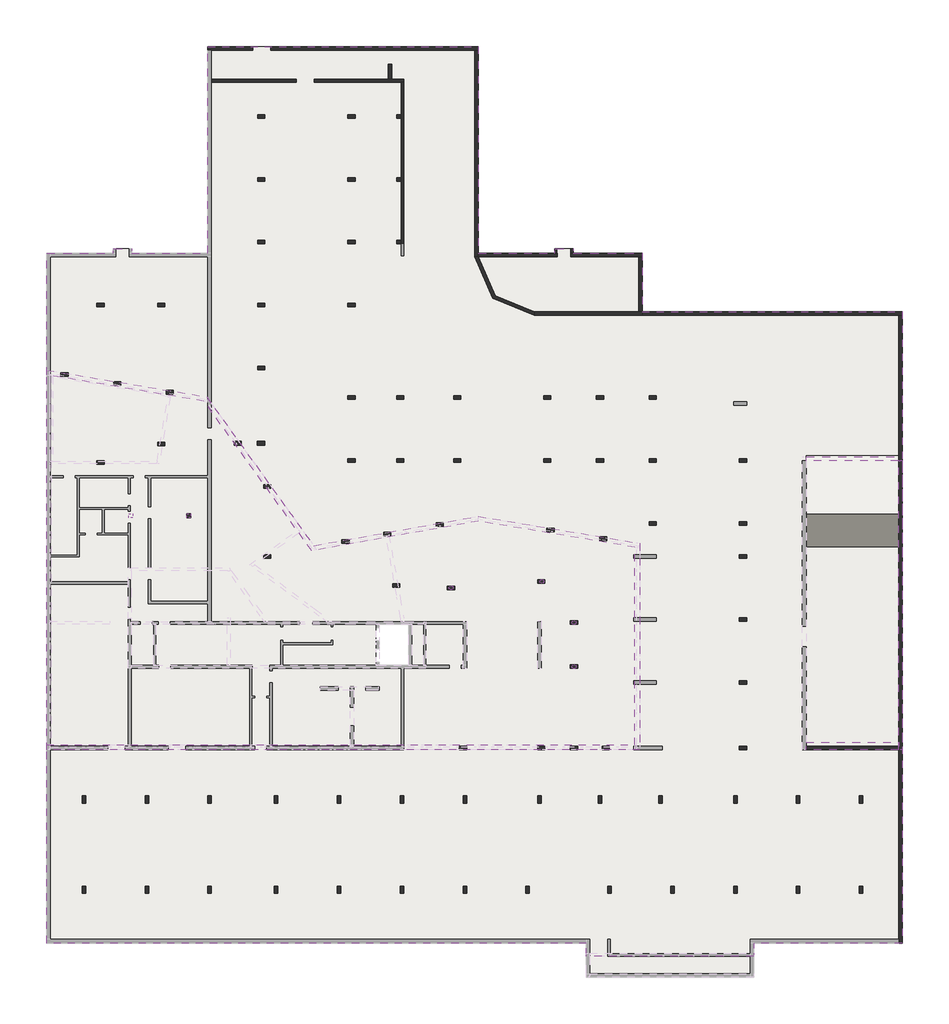
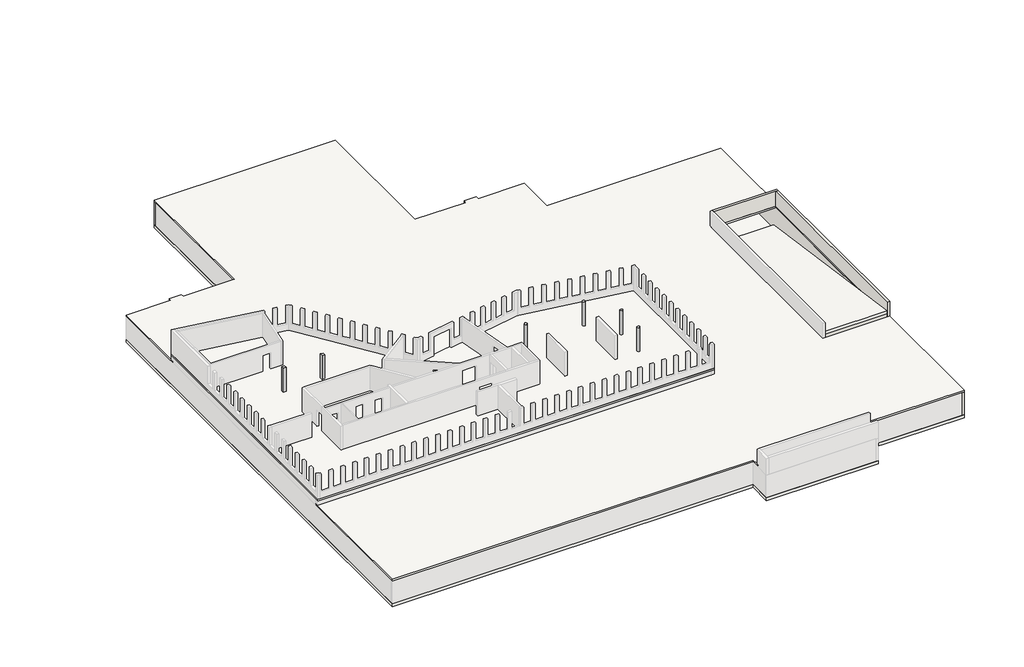
# One storey, part 4 of 4: 89 columns, 17 walls, 4 slabs.
"""IFC4 building model written with IfcOpenShell, lengths in millimetres."""

import ifcopenshell
import ifcopenshell.guid

model = None  # the IFC model being written
_history = None  # IfcOwnerHistory: only IFC2X3 demands one
_inside = {}  # id of a spatial element -> (the spatial element, [elements in it])
_under = {}  # id of a project, library or spatial element -> (it, [spatial elements below it])
_declared = {}  # id of a project -> (the project, [libraries it declares])
_typed = {}  # id of a type object -> (the type object, [elements of that type])
_made_of = {}  # id of a material, layer set ... -> (it, [elements and type objects made of it])


def new_model(schema):
    """Start an empty IFC model of exactly this schema.

    Asked for "IFC4X3", IfcOpenShell would pick the latest addendum, in which some entities
    have other attributes; the version numbers below select the first issue.
    IFC2X3 requires an IfcOwnerHistory on every rooted entity: one is made here for all.
    """
    global model, _history
    if schema == "IFC4X3":
        model = ifcopenshell.file(schema_version=(4, 3, 0, 0))
    else:
        model = ifcopenshell.file(schema=schema)
    _inside.clear()
    _under.clear()
    _declared.clear()
    _typed.clear()
    _made_of.clear()
    _history = None
    if model.schema == "IFC2X3":
        org = make("IfcOrganization", Name="unknown")
        user = make(
            "IfcPersonAndOrganization",
            ThePerson=make("IfcPerson", FamilyName="unknown"),
            TheOrganization=org,
        )
        app = make(
            "IfcApplication",
            ApplicationDeveloper=org,
            Version="unknown",
            ApplicationFullName="unknown",
            ApplicationIdentifier="unknown",
        )
        _history = make(
            "IfcOwnerHistory",
            OwningUser=user,
            OwningApplication=app,
            ChangeAction="ADDED",
            CreationDate=0,
        )
    return model


def make(cls, **values):
    """One entity of the class cls with the attributes given. An attribute that is None is left unset."""
    return model.create_entity(
        cls, **{name: value for name, value in values.items() if value is not None}
    )


def rooted(cls, **values):
    """An entity with a GlobalId (a new one), such as an element, a storey or a relation."""
    return make(cls, GlobalId=ifcopenshell.guid.new(), OwnerHistory=_history, **values)


def si_unit(unit_type, name, prefix=None):
    """IfcSIUnit, for example si_unit("LENGTHUNIT", "METRE", prefix="MILLI")."""
    return make("IfcSIUnit", UnitType=unit_type, Prefix=prefix, Name=name)


def assignment(units):
    """IfcUnitAssignment: the units of a project."""
    return None if units is None else make("IfcUnitAssignment", Units=units)


def point(xyz):
    """IfcCartesianPoint."""
    return None if xyz is None else make("IfcCartesianPoint", Coordinates=xyz)


def direction(xyz):
    """IfcDirection."""
    return None if xyz is None else make("IfcDirection", DirectionRatios=xyz)


def frame(location, z_axis=None, x_axis=None):
    """IfcAxis2Placement3D, a coordinate frame: its origin and axes. An axis left out is left unset."""
    return make(
        "IfcAxis2Placement3D",
        Location=point(location),
        Axis=direction(z_axis),
        RefDirection=direction(x_axis),
    )


def frame_2d(location, x_axis=None):
    """IfcAxis2Placement2D, a coordinate frame in the plane: its origin and x axis."""
    return make(
        "IfcAxis2Placement2D", Location=point(location), RefDirection=direction(x_axis)
    )


def origin():
    """The frame at (0, 0, 0) with its axes left unset."""
    return frame((0.0, 0.0, 0.0))


def place(relative_to, where):
    """IfcLocalPlacement: puts the frame where relative to a parent placement (None: the world)."""
    return make(
        "IfcLocalPlacement", PlacementRelTo=relative_to, RelativePlacement=where
    )


def context(
    kind, dimensions, precision=None, world=None, true_north=None, identifier=None
):
    """IfcGeometricRepresentationContext, for example the 3D "Model" context."""
    return make(
        "IfcGeometricRepresentationContext",
        ContextIdentifier=identifier,
        ContextType=kind,
        CoordinateSpaceDimension=dimensions,
        Precision=precision,
        WorldCoordinateSystem=world,
        TrueNorth=true_north,
    )


def project(units=None, contexts=None):
    """IfcProject with its units and contexts."""
    return rooted(
        "IfcProject",
        Name="project",
        RepresentationContexts=contexts,
        UnitsInContext=assignment(units),
    )


def spatial(cls, under=None, at=None, **own):
    """A site, building, storey or space (cls), placed at a placement, below another one or the project."""
    s = rooted(cls, ObjectPlacement=at, **own)
    if under is not None:
        _under.setdefault(under.id(), (under, []))[1].append(s)
    return s


def polyline(points):
    """IfcPolyline through the points."""
    return make("IfcPolyline", Points=[point(p) for p in points])


def circle_curve(where, radius):
    """IfcCircle in the frame where."""
    return make("IfcCircle", Position=where, Radius=radius)


def trimmed(basis, trim1, trim2, sense, master):
    """IfcTrimmedCurve: the piece of a basis curve between two trims."""
    return make(
        "IfcTrimmedCurve",
        BasisCurve=basis,
        Trim1=trim1,
        Trim2=trim2,
        SenseAgreement=sense,
        MasterRepresentation=master,
    )


def segment(curve, same_sense, transition):
    """IfcCompositeCurveSegment."""
    return make(
        "IfcCompositeCurveSegment",
        Transition=transition,
        SameSense=same_sense,
        ParentCurve=curve,
    )


def composite_curve(segments, self_intersect=None):
    """IfcCompositeCurve: segments joined end to end."""
    return make("IfcCompositeCurve", Segments=segments, SelfIntersect=self_intersect)


def outline(outer, holes=None, kind="AREA"):
    """IfcArbitraryClosedProfileDef: a profile drawn as a closed curve; with holes, ...WithVoids."""
    if holes is None:
        return make("IfcArbitraryClosedProfileDef", ProfileType=kind, OuterCurve=outer)
    return make(
        "IfcArbitraryProfileDefWithVoids",
        ProfileType=kind,
        OuterCurve=outer,
        InnerCurves=holes,
    )


def extrude(swept, where, along, depth):
    """IfcExtrudedAreaSolid: the profile swept, set in the frame where, extruded along a direction by depth."""
    return make(
        "IfcExtrudedAreaSolid",
        SweptArea=swept,
        Position=where,
        ExtrudedDirection=direction(along),
        Depth=depth,
    )


def faces_of(points, faces, orient=None, outer=None):
    """IfcFace entities. A face is a list of loops; a loop is a list of indices into points, from 0.

    orient and outer hold one flag for each loop. By default every Orientation is true, the
    first loop of a face is its IfcFaceOuterBound and the others are IfcFaceBound.
    """
    made = []
    for i, loops in enumerate(faces):
        bounds = []
        for j, loop in enumerate(loops):
            is_outer = j == 0 if outer is None else outer[i][j]
            bounds.append(
                make(
                    "IfcFaceOuterBound" if is_outer else "IfcFaceBound",
                    Bound=make("IfcPolyLoop", Polygon=[points[k] for k in loop]),
                    Orientation=True if orient is None else orient[i][j],
                )
            )
        made.append(make("IfcFace", Bounds=bounds))
    return made


def faceted_brep(points, faces, orient=None, outer=None, voids=None):
    """IfcFacetedBrep: a solid bounded by flat faces; with voids (closed shells), ...WithVoids."""
    shared = [point(p) for p in points]
    hull = make("IfcClosedShell", CfsFaces=faces_of(shared, faces, orient, outer))
    if voids is None:
        return make("IfcFacetedBrep", Outer=hull)
    return make(
        "IfcFacetedBrepWithVoids",
        Outer=hull,
        Voids=[
            make(cls, CfsFaces=faces_of(shared, fs, o, b)) for cls, fs, o, b in voids
        ],
    )


def shape(context_of_items, identifier, shape_type, items):
    """IfcShapeRepresentation: the items that make up one representation, for example the "Body"."""
    return make(
        "IfcShapeRepresentation",
        ContextOfItems=context_of_items,
        RepresentationIdentifier=identifier,
        RepresentationType=shape_type,
        Items=items,
    )


def source(mapping_origin, context_of_items, identifier, shape_type, items):
    """IfcRepresentationMap: a shape defined once, which mapped items show again and again."""
    return make(
        "IfcRepresentationMap",
        MappingOrigin=mapping_origin,
        MappedRepresentation=shape(context_of_items, identifier, shape_type, items),
    )


def transform(
    local_origin,
    x_axis=None,
    y_axis=None,
    z_axis=None,
    scale=None,
    scale2=None,
    scale3=None,
    uniform=True,
):
    """IfcCartesianTransformationOperator3D, or its non-uniform kind. x_axis, y_axis, z_axis: its Axis1, 2, 3."""
    if uniform:
        return make(
            "IfcCartesianTransformationOperator3D",
            Axis1=direction(x_axis),
            Axis2=direction(y_axis),
            LocalOrigin=point(local_origin),
            Scale=scale,
            Axis3=direction(z_axis),
        )
    return make(
        "IfcCartesianTransformationOperator3DnonUniform",
        Axis1=direction(x_axis),
        Axis2=direction(y_axis),
        LocalOrigin=point(local_origin),
        Scale=scale,
        Axis3=direction(z_axis),
        Scale2=scale2,
        Scale3=scale3,
    )


def mapped(mapping_source, mapping_target):
    """IfcMappedItem: shows the shape of a source again, moved by a transform."""
    return make(
        "IfcMappedItem", MappingSource=mapping_source, MappingTarget=mapping_target
    )


def made_of(thing, what):
    """Note that an element or type object is made of a material, layer set ...; save() writes the relation."""
    if what is not None:
        _made_of.setdefault(what.id(), (what, []))[1].append(thing)
    return thing


def element(
    cls,
    number,
    at=None,
    inside=None,
    cuts=None,
    type_object=None,
    material=None,
    context=None,
    identifier="Body",
    shape_type=None,
    held_by="IfcProductDefinitionShape",
    body=None,
    shapes=None,
    **own,
):
    """One element of the class cls, such as IfcWall. Its Tag is "e" and its number.

    at: its placement. inside: the storey or other place that contains it. cuts: it is an
    opening in that element (IfcRelVoidsElement). A single representation is given by context,
    identifier, shape_type and body (its items); several are given by shapes. held_by: the class
    of the entity that holds the representations. save() writes the other relations.
    """
    e = rooted(cls, Tag="e%d" % number, ObjectPlacement=at, **own)
    if body is not None:
        shapes = [shape(context, identifier, shape_type, body)]
    if shapes is not None:
        e.Representation = make(held_by, Representations=shapes)
    if inside is not None:
        _inside.setdefault(inside.id(), (inside, []))[1].append(e)
    if cuts is not None:
        rooted(
            "IfcRelVoidsElement", RelatingBuildingElement=cuts, RelatedOpeningElement=e
        )
    if type_object is not None:
        _typed.setdefault(type_object.id(), (type_object, []))[1].append(e)
    return made_of(e, material)


def aggregate(whole, parts):
    """IfcRelAggregates: a whole, such as a stair, and the parts it consists of."""
    return rooted("IfcRelAggregates", RelatingObject=whole, RelatedObjects=parts)


def save(model, path):
    """Write the relations noted so far, then the file.

    IfcRelAggregates (storeys below a building ...), IfcRelContainedInSpatialStructure (elements
    in a storey), IfcRelDefinesByType, IfcRelAssociatesMaterial and IfcRelDeclares: one each for
    every whole, place, type object, material and project.
    """
    for whole, parts in _under.values():
        aggregate(whole, parts)
    for where, things in _inside.values():
        rooted(
            "IfcRelContainedInSpatialStructure",
            RelatedElements=things,
            RelatingStructure=where,
        )
    for kind, things in _typed.values():
        rooted("IfcRelDefinesByType", RelatedObjects=things, RelatingType=kind)
    for what, things in _made_of.values():
        rooted("IfcRelAssociatesMaterial", RelatedObjects=things, RelatingMaterial=what)
    for by, libraries in _declared.values():
        rooted("IfcRelDeclares", RelatingContext=by, RelatedDefinitions=libraries)
    model.write(path)


def column_b848c13c(model_context):
    return source(origin(), model_context, "Body", "SweptSolid", [
        extrude(outline(polyline([(300.0, 150.0), (300.0, -150.0), (-300.0, -150.0), (-300.0, 150.0), (300.0, 150.0)])), frame((0.0, 0.0, -4200.0), z_axis=(0.0, 0.0, 1.0), x_axis=(1.0, 0.0, 0.0)), (0.0, 0.0, 1.0), 3000.0),
    ])


model = new_model("IFC4")

# Units and contexts
model_context = context("Model", 3, world=origin())
ifc_project = project(units=[si_unit("LENGTHUNIT", "METRE", prefix="MILLI")], contexts=[model_context])

# Site, building, storey
site = spatial("IfcSite", under=ifc_project)
building = spatial("IfcBuilding", under=site)
storey = spatial("IfcBuildingStorey", under=building, Name="01_UG_OKFB_-4,20", Elevation=-4200.0)

# Columns
placement = place(None, origin())
element("IfcColumn", 1, at=placement, inside=storey, context=model_context, shape_type="SweptSolid", body=[
    extrude(outline(composite_curve([segment(trimmed(circle_curve(frame_2d((33961.7583834, 13503.0230367)), 175.0), [point((34136.7583834, 13503.0230367))], [point((33786.7583834, 13503.0230367))], False, "CARTESIAN"), True, "CONTINUOUS"), segment(trimmed(circle_curve(frame_2d((33961.7583834, 13503.0230367)), 175.0), [point((33786.7583834, 13503.0230367))], [point((34136.7583834, 13503.0230367))], False, "CARTESIAN"), True, "CONTINUOUS")], self_intersect=False)), frame((0.0, 0.0, -150.0), z_axis=(0.0, 0.0, 1.0), x_axis=(1.0, 0.0, 0.0)), (0.0, 0.0, 1.0), 3210.0),
])
element("IfcColumn", 2, at=placement, inside=storey, context=model_context, shape_type="SweptSolid", body=[
    extrude(outline(polyline([(7139.9999521, 19742.0124565), (7139.9999521, 19392.0124565), (6789.9999521, 19392.0124565), (6789.9999521, 19742.0124565), (7139.9999521, 19742.0124565)])), frame((0.0, 0.0, -150.0), z_axis=(0.0, 0.0, 1.0), x_axis=(1.0, 0.0, 0.0)), (0.0, 0.0, 1.0), 3210.0),
])
element("IfcColumn", 3, at=placement, inside=storey, context=model_context, shape_type="SweptSolid", body=[
    extrude(outline(polyline([(12021.4450432, 19742.0124565), (12021.4450432, 19392.0124565), (11671.4450432, 19392.0124565), (11671.4450432, 19742.0124565), (12021.4450432, 19742.0124565)])), frame((0.0, 0.0, -150.0), z_axis=(0.0, 0.0, 1.0), x_axis=(1.0, 0.0, 0.0)), (0.0, 0.0, 1.0), 3210.0),
])
element("IfcColumn", 4, at=placement, inside=storey, context=model_context, shape_type="SweptSolid", body=[
    extrude(outline(composite_curve([segment(trimmed(circle_curve(frame_2d((41616.0718251, 14052.9332427)), 175.0), [point((41791.0718251, 14052.9332427))], [point((41441.0718251, 14052.9332427))], False, "CARTESIAN"), True, "CONTINUOUS"), segment(trimmed(circle_curve(frame_2d((41616.0718251, 14052.9332427)), 175.0), [point((41441.0718251, 14052.9332427))], [point((41791.0718251, 14052.9332427))], False, "CARTESIAN"), True, "CONTINUOUS")], self_intersect=False)), frame((0.0, 0.0, -150.0), z_axis=(0.0, 0.0, 1.0), x_axis=(1.0, 0.0, 0.0)), (0.0, 0.0, 1.0), 3210.0),
])
element("IfcColumn", 5, at=placement, inside=storey, context=model_context, shape_type="SweptSolid", body=[
    extrude(outline(composite_curve([segment(trimmed(circle_curve(frame_2d((44328.9990923, 10566.8309986)), 175.0), [point((44503.9990923, 10566.8309986))], [point((44153.9990923, 10566.8309986))], False, "CARTESIAN"), True, "CONTINUOUS"), segment(trimmed(circle_curve(frame_2d((44328.9990923, 10566.8309986)), 175.0), [point((44153.9990923, 10566.8309986))], [point((44503.9990923, 10566.8309986))], False, "CARTESIAN"), True, "CONTINUOUS")], self_intersect=False)), frame((0.0, 0.0, -150.0), z_axis=(0.0, 0.0, 1.0), x_axis=(1.0, 0.0, 0.0)), (0.0, 0.0, 1.0), 3210.0),
])
element("IfcColumn", 6, at=placement, inside=storey, context=model_context, shape_type="SweptSolid", body=[
    extrude(outline(composite_curve([segment(trimmed(circle_curve(frame_2d((44328.9990923, 6852.1619165)), 175.0), [point((44503.9990923, 6852.1619165))], [point((44153.9990923, 6852.1619165))], False, "CARTESIAN"), True, "CONTINUOUS"), segment(trimmed(circle_curve(frame_2d((44328.9990923, 6852.1619165)), 175.0), [point((44153.9990923, 6852.1619165))], [point((44503.9990923, 6852.1619165))], False, "CARTESIAN"), True, "CONTINUOUS")], self_intersect=False)), frame((0.0, 0.0, -150.0), z_axis=(0.0, 0.0, 1.0), x_axis=(1.0, 0.0, 0.0)), (0.0, 0.0, 1.0), 3210.0),
])
element("IfcColumn", 7, at=placement, inside=storey, context=model_context, shape_type="SweptSolid", body=[
    extrude(outline(polyline([(29370.0001853, 47785.5744998), (29370.0001853, 48085.5744998), (29770.0002004, 48085.5744998), (29770.0001932, 47785.5744998), (29370.0001853, 47785.5744998)])), frame((0.0, 0.0, -4200.0), z_axis=(0.0, 0.0, 1.0), x_axis=(1.0, 0.0, 0.0)), (0.0, 0.0, 1.0), 3000.0),
])
element("IfcColumn", 8, at=placement, inside=storey, context=model_context, shape_type="SweptSolid", body=[
    extrude(outline(polyline([(29370.00024, 53085.5744986), (29370.00024, 53385.5744986), (29770.0003285, 53385.5744986), (29770.0003212, 53085.5744986), (29370.00024, 53085.5744986)])), frame((0.0, 0.0, -4200.0), z_axis=(0.0, 0.0, 1.0), x_axis=(1.0, 0.0, 0.0)), (0.0, 0.0, 1.0), 3000.0),
])
element("IfcColumn", 9, at=placement, inside=storey, context=model_context, shape_type="SweptSolid", body=[
    extrude(outline(polyline([(29370.0000575, 42485.5744993), (29370.0000575, 42785.5744993), (29770.0000724, 42785.5744993), (29770.0000651, 42485.5744993), (29370.0000575, 42485.5744993)])), frame((0.0, 0.0, -4200.0), z_axis=(0.0, 0.0, 1.0), x_axis=(1.0, 0.0, 0.0)), (0.0, 0.0, 1.0), 3000.0),
])
element("IfcColumn", 10, at=placement, inside=storey, context=model_context, shape_type="SweptSolid", body=[
    extrude(outline(polyline([(12021.8084323, 19742.0126094), (12021.8084323, 19392.0126094), (11671.8084323, 19392.0126094), (11671.8084323, 19742.0126094), (12021.8084323, 19742.0126094)])), frame((0.0, 0.0, -4200.0), z_axis=(0.0, 0.0, 1.0), x_axis=(1.0, 0.0, 0.0)), (0.0, 0.0, 1.0), 3000.0),
])
column_shape = column_b848c13c(model_context)
element("IfcColumn", 11, at=placement, inside=storey, context=model_context, shape_type="MappedRepresentation", body=[
    mapped(column_shape, transform((17970.0003295, 53235.5747843, 0.0), x_axis=(1.0, 0.0, 0.0), y_axis=(0.0, 1.0, 0.0), z_axis=(0.0, 0.0, 1.0))),
])
element("IfcColumn", 12, at=placement, inside=storey, context=model_context, shape_type="MappedRepresentation", body=[
    mapped(column_shape, transform((25570.0002271, 53235.5745978, 0.0), x_axis=(1.0, 0.0, 0.0), y_axis=(0.0, 1.0, 0.0), z_axis=(0.0, 0.0, 1.0))),
])
element("IfcColumn", 13, at=placement, inside=storey, context=model_context, shape_type="MappedRepresentation", body=[
    mapped(column_shape, transform((25570.0000997, 47935.5745982, 0.0), x_axis=(1.0, 0.0, 0.0), y_axis=(0.0, 1.0, 0.0), z_axis=(0.0, 0.0, 1.0))),
])
element("IfcColumn", 14, at=placement, inside=storey, context=model_context, shape_type="MappedRepresentation", body=[
    mapped(column_shape, transform((17970.0001541, 47935.5747703, 0.0), x_axis=(1.0, 0.0, 0.0), y_axis=(0.0, 1.0, 0.0), z_axis=(0.0, 0.0, 1.0))),
])
element("IfcColumn", 15, at=placement, inside=storey, context=model_context, shape_type="MappedRepresentation", body=[
    mapped(column_shape, transform((17970.0000672, 42635.5747706, 0.0), x_axis=(1.0, 0.0, 0.0), y_axis=(0.0, 1.0, 0.0), z_axis=(0.0, 0.0, 1.0))),
])
element("IfcColumn", 16, at=placement, inside=storey, context=model_context, shape_type="MappedRepresentation", body=[
    mapped(column_shape, transform((25569.9999727, 42635.5745841, 0.0), x_axis=(1.0, 0.0, 0.0), y_axis=(0.0, 1.0, 0.0), z_axis=(0.0, 0.0, 1.0))),
])
element("IfcColumn", 17, at=placement, inside=storey, context=model_context, shape_type="MappedRepresentation", body=[
    mapped(column_shape, transform((25569.9998415, 37335.5745988, 0.0), x_axis=(1.0, 0.0, 0.0), y_axis=(0.0, 1.0, 0.0), z_axis=(0.0, 0.0, 1.0))),
])
element("IfcColumn", 18, at=placement, inside=storey, context=model_context, shape_type="MappedRepresentation", body=[
    mapped(column_shape, transform((17969.999937, 37335.5747853, 0.0), x_axis=(1.0, 0.0, 0.0), y_axis=(0.0, 1.0, 0.0), z_axis=(0.0, 0.0, 1.0))),
])
element("IfcColumn", 19, at=placement, inside=storey, context=model_context, shape_type="MappedRepresentation", body=[
    mapped(column_shape, transform((3019.9989244, -4329.9988646, 0.0), x_axis=(0.0, -1.0, 0.0), y_axis=(1.0, 0.0, 0.0), z_axis=(0.0, 0.0, 1.0))),
])
element("IfcColumn", 20, at=placement, inside=storey, context=model_context, shape_type="MappedRepresentation", body=[
    mapped(column_shape, transform((8319.9989229, -4329.9989954, 0.0), x_axis=(0.0, -1.0, 0.0), y_axis=(1.0, 0.0, 0.0), z_axis=(0.0, 0.0, 1.0))),
])
element("IfcColumn", 21, at=placement, inside=storey, context=model_context, shape_type="MappedRepresentation", body=[
    mapped(column_shape, transform((13619.9989086, -4329.9991251, 0.0), x_axis=(0.0, -1.0, 0.0), y_axis=(1.0, 0.0, 0.0), z_axis=(0.0, 0.0, 1.0))),
])
element("IfcColumn", 22, at=placement, inside=storey, context=model_context, shape_type="MappedRepresentation", body=[
    mapped(column_shape, transform((19219.9989245, -4329.9992634, 0.0), x_axis=(0.0, -1.0, 0.0), y_axis=(1.0, 0.0, 0.0), z_axis=(0.0, 0.0, 1.0))),
])
element("IfcColumn", 23, at=placement, inside=storey, context=model_context, shape_type="MappedRepresentation", body=[
    mapped(column_shape, transform((3019.9987398, -11929.998882, 0.0), x_axis=(0.0, -1.0, 0.0), y_axis=(1.0, 0.0, 0.0), z_axis=(0.0, 0.0, 1.0))),
])
element("IfcColumn", 24, at=placement, inside=storey, context=model_context, shape_type="MappedRepresentation", body=[
    mapped(column_shape, transform((24519.9989228, -4329.9993595, 0.0), x_axis=(0.0, -1.0, 0.0), y_axis=(1.0, 0.0, 0.0), z_axis=(0.0, 0.0, 1.0))),
])
element("IfcColumn", 25, at=placement, inside=storey, context=model_context, shape_type="MappedRepresentation", body=[
    mapped(column_shape, transform((24519.9987381, -11929.9993769, 0.0), x_axis=(0.0, -1.0, 0.0), y_axis=(1.0, 0.0, 0.0), z_axis=(0.0, 0.0, 1.0))),
])
element("IfcColumn", 26, at=placement, inside=storey, context=model_context, shape_type="MappedRepresentation", body=[
    mapped(column_shape, transform((29819.9989229, -4329.9994883, 0.0), x_axis=(0.0, -1.0, 0.0), y_axis=(1.0, 0.0, 0.0), z_axis=(0.0, 0.0, 1.0))),
])
element("IfcColumn", 27, at=placement, inside=storey, context=model_context, shape_type="MappedRepresentation", body=[
    mapped(column_shape, transform((29819.9987383, -11929.9995057, 0.0), x_axis=(0.0, -1.0, 0.0), y_axis=(1.0, 0.0, 0.0), z_axis=(0.0, 0.0, 1.0))),
])
element("IfcColumn", 28, at=placement, inside=storey, context=model_context, shape_type="MappedRepresentation", body=[
    mapped(column_shape, transform((35119.9989224, -4329.99962, 0.0), x_axis=(0.0, -1.0, 0.0), y_axis=(1.0, 0.0, 0.0), z_axis=(0.0, 0.0, 1.0))),
])
element("IfcColumn", 29, at=placement, inside=storey, context=model_context, shape_type="MappedRepresentation", body=[
    mapped(column_shape, transform((35119.9987378, -11929.9996374, 0.0), x_axis=(0.0, -1.0, 0.0), y_axis=(1.0, 0.0, 0.0), z_axis=(0.0, 0.0, 1.0))),
])
element("IfcColumn", 30, at=placement, inside=storey, context=model_context, shape_type="MappedRepresentation", body=[
    mapped(column_shape, transform((41400.9133491, -4329.9997741, 0.0), x_axis=(0.0, -1.0, 0.0), y_axis=(1.0, 0.0, 0.0), z_axis=(0.0, 0.0, 1.0))),
])
element("IfcColumn", 31, at=placement, inside=storey, context=model_context, shape_type="MappedRepresentation", body=[
    mapped(column_shape, transform((46500.9133631, -4329.9998991, 0.0), x_axis=(0.0, -1.0, 0.0), y_axis=(1.0, 0.0, 0.0), z_axis=(0.0, 0.0, 1.0))),
])
element("IfcColumn", 32, at=placement, inside=storey, context=model_context, shape_type="MappedRepresentation", body=[
    mapped(column_shape, transform((51600.9131437, -4330.0000246, 0.0), x_axis=(0.0, -1.0, 0.0), y_axis=(1.0, 0.0, 0.0), z_axis=(0.0, 0.0, 1.0))),
])
element("IfcColumn", 33, at=placement, inside=storey, context=model_context, shape_type="MappedRepresentation", body=[
    mapped(column_shape, transform((57919.9989252, -4330.0002007, 0.0), x_axis=(0.0, -1.0, 0.0), y_axis=(1.0, 0.0, 0.0), z_axis=(0.0, 0.0, 1.0))),
])
element("IfcColumn", 34, at=placement, inside=storey, context=model_context, shape_type="MappedRepresentation", body=[
    mapped(column_shape, transform((63219.9989396, -4330.000302, 0.0), x_axis=(0.0, -1.0, 0.0), y_axis=(1.0, 0.0, 0.0), z_axis=(0.0, 0.0, 1.0))),
])
element("IfcColumn", 35, at=placement, inside=storey, context=model_context, shape_type="MappedRepresentation", body=[
    mapped(column_shape, transform((68519.9989422, -4330.0003933, 0.0), x_axis=(0.0, -1.0, 0.0), y_axis=(1.0, 0.0, 0.0), z_axis=(0.0, 0.0, 1.0))),
])
element("IfcColumn", 36, at=placement, inside=storey, context=model_context, shape_type="MappedRepresentation", body=[
    mapped(column_shape, transform((68519.9987395, -11930.0004072, 0.0), x_axis=(0.0, -1.0, 0.0), y_axis=(1.0, 0.0, 0.0), z_axis=(0.0, 0.0, 1.0))),
])
element("IfcColumn", 37, at=placement, inside=storey, context=model_context, shape_type="MappedRepresentation", body=[
    mapped(column_shape, transform((63219.9987395, -11930.0004072, 0.0), x_axis=(0.0, -1.0, 0.0), y_axis=(1.0, 0.0, 0.0), z_axis=(0.0, 0.0, 1.0))),
])
element("IfcColumn", 38, at=placement, inside=storey, context=model_context, shape_type="MappedRepresentation", body=[
    mapped(column_shape, transform((57919.9987396, -11930.0001978, 0.0), x_axis=(0.0, -1.0, 0.0), y_axis=(1.0, 0.0, 0.0), z_axis=(0.0, 0.0, 1.0))),
])
element("IfcColumn", 39, at=placement, inside=storey, context=model_context, shape_type="MappedRepresentation", body=[
    mapped(column_shape, transform((52619.9987394, -11930.0000615, 0.0), x_axis=(0.0, -1.0, 0.0), y_axis=(1.0, 0.0, 0.0), z_axis=(0.0, 0.0, 1.0))),
])
element("IfcColumn", 40, at=placement, inside=storey, context=model_context, shape_type="MappedRepresentation", body=[
    mapped(column_shape, transform((47319.9987533, -11929.9999328, 0.0), x_axis=(0.0, -1.0, 0.0), y_axis=(1.0, 0.0, 0.0), z_axis=(0.0, 0.0, 1.0))),
])
element("IfcColumn", 41, at=placement, inside=storey, context=model_context, shape_type="MappedRepresentation", body=[
    mapped(column_shape, transform((40419.9987404, -11929.9997669, 0.0), x_axis=(0.0, -1.0, 0.0), y_axis=(1.0, 0.0, 0.0), z_axis=(0.0, 0.0, 1.0))),
])
element("IfcColumn", 42, at=placement, inside=storey, context=model_context, shape_type="MappedRepresentation", body=[
    mapped(column_shape, transform((19219.9987539, -11929.999248, 0.0), x_axis=(0.0, -1.0, 0.0), y_axis=(1.0, 0.0, 0.0), z_axis=(0.0, 0.0, 1.0))),
])
element("IfcColumn", 43, at=placement, inside=storey, context=model_context, shape_type="MappedRepresentation", body=[
    mapped(column_shape, transform((13619.9987548, -11929.9991263, 0.0), x_axis=(0.0, -1.0, 0.0), y_axis=(1.0, 0.0, 0.0), z_axis=(0.0, 0.0, 1.0))),
])
element("IfcColumn", 44, at=placement, inside=storey, context=model_context, shape_type="MappedRepresentation", body=[
    mapped(column_shape, transform((8319.9987398, -11929.9990003, 0.0), x_axis=(0.0, -1.0, 0.0), y_axis=(1.0, 0.0, 0.0), z_axis=(0.0, 0.0, 1.0))),
])
element("IfcColumn", 45, at=placement, inside=storey, context=model_context, shape_type="MappedRepresentation", body=[
    mapped(column_shape, transform((4416.9998447, 37335.5751137, 0.0), x_axis=(1.0, 0.0, 0.0), y_axis=(0.0, 1.0, 0.0), z_axis=(0.0, 0.0, 1.0))),
])
element("IfcColumn", 46, at=placement, inside=storey, context=model_context, shape_type="MappedRepresentation", body=[
    mapped(column_shape, transform((9535.2709352, 37335.5749769, 0.0), x_axis=(1.0, 0.0, 0.0), y_axis=(0.0, 1.0, 0.0), z_axis=(0.0, 0.0, 1.0))),
])
element("IfcColumn", 47, at=placement, inside=storey, context=model_context, shape_type="MappedRepresentation", body=[
    mapped(column_shape, transform((10260.9910129, 29989.0471188, 0.0), x_axis=(1.0, 0.0, 0.0), y_axis=(0.0, 1.0, 0.0), z_axis=(0.0, 0.0, 1.0))),
])
element("IfcColumn", 48, at=placement, inside=storey, context=model_context, shape_type="MappedRepresentation", body=[
    mapped(column_shape, transform((5822.7557859, 30729.5383476, 0.0), x_axis=(1.0, 0.0, 0.0), y_axis=(0.0, 1.0, 0.0), z_axis=(0.0, 0.0, 1.0))),
])
element("IfcColumn", 49, at=placement, inside=storey, context=model_context, shape_type="MappedRepresentation", body=[
    mapped(column_shape, transform((1384.4105374, 31470.7182326, 0.0), x_axis=(1.0, 0.0, 0.0), y_axis=(0.0, 1.0, 0.0), z_axis=(0.0, 0.0, 1.0))),
])
element("IfcColumn", 50, at=placement, inside=storey, context=model_context, shape_type="MappedRepresentation", body=[
    mapped(column_shape, transform((4416.9995228, 24067.0135892, 0.0), x_axis=(1.0, 0.0, 0.0), y_axis=(0.0, 1.0, 0.0), z_axis=(0.0, 0.0, 1.0))),
])
element("IfcColumn", 51, at=placement, inside=storey, context=model_context, shape_type="MappedRepresentation", body=[
    mapped(column_shape, transform((18469.9994281, 16135.5747249, 0.0), x_axis=(1.0, 0.0, 0.0), y_axis=(0.0, 1.0, 0.0), z_axis=(0.0, 0.0, 1.0))),
])
element("IfcColumn", 52, at=placement, inside=storey, context=model_context, shape_type="MappedRepresentation", body=[
    mapped(column_shape, transform((18469.9994743, 22040.8888187, 0.0), x_axis=(1.0, 0.0, 0.0), y_axis=(0.0, 1.0, 0.0), z_axis=(0.0, 0.0, 1.0))),
])
element("IfcColumn", 53, at=placement, inside=storey, context=model_context, shape_type="MappedRepresentation", body=[
    mapped(column_shape, transform((17940.8526488, 25691.6484492, 0.0), x_axis=(1.0, 0.0, 0.0), y_axis=(0.0, 1.0, 0.0), z_axis=(0.0, 0.0, 1.0))),
])
element("IfcColumn", 54, at=placement, inside=storey, context=model_context, shape_type="MappedRepresentation", body=[
    mapped(column_shape, transform((15985.3006928, 25691.6484935, 0.0), x_axis=(1.0, 0.0, 0.0), y_axis=(0.0, 1.0, 0.0), z_axis=(0.0, 0.0, 1.0))),
])
element("IfcColumn", 55, at=placement, inside=storey, context=model_context, shape_type="MappedRepresentation", body=[
    mapped(column_shape, transform((25569.9996255, 24235.5745998, 0.0), x_axis=(1.0, 0.0, 0.0), y_axis=(0.0, 1.0, 0.0), z_axis=(0.0, 0.0, 1.0))),
])
element("IfcColumn", 56, at=placement, inside=storey, context=model_context, shape_type="MappedRepresentation", body=[
    mapped(column_shape, transform((29670.000239, 24235.5744956, 0.0), x_axis=(1.0, 0.0, 0.0), y_axis=(0.0, 1.0, 0.0), z_axis=(0.0, 0.0, 1.0))),
])
element("IfcColumn", 57, at=placement, inside=storey, context=model_context, shape_type="MappedRepresentation", body=[
    mapped(column_shape, transform((25569.9997505, 29535.5746011, 0.0), x_axis=(1.0, 0.0, 0.0), y_axis=(0.0, 1.0, 0.0), z_axis=(0.0, 0.0, 1.0))),
])
element("IfcColumn", 58, at=placement, inside=storey, context=model_context, shape_type="MappedRepresentation", body=[
    mapped(column_shape, transform((29670.0003655, 29535.5744807, 0.0), x_axis=(1.0, 0.0, 0.0), y_axis=(0.0, 1.0, 0.0), z_axis=(0.0, 0.0, 1.0))),
])
element("IfcColumn", 59, at=placement, inside=storey, context=model_context, shape_type="MappedRepresentation", body=[
    mapped(column_shape, transform((34469.9997526, 29535.5743843, 0.0), x_axis=(1.0, 0.0, 0.0), y_axis=(0.0, 1.0, 0.0), z_axis=(0.0, 0.0, 1.0))),
])
element("IfcColumn", 60, at=placement, inside=storey, context=model_context, shape_type="MappedRepresentation", body=[
    mapped(column_shape, transform((42069.9997513, 29535.5741866, 0.0), x_axis=(1.0, 0.0, 0.0), y_axis=(0.0, 1.0, 0.0), z_axis=(0.0, 0.0, 1.0))),
])
element("IfcColumn", 61, at=placement, inside=storey, context=model_context, shape_type="MappedRepresentation", body=[
    mapped(column_shape, transform((46519.9997529, 29535.5740801, 0.0), x_axis=(1.0, 0.0, 0.0), y_axis=(0.0, 1.0, 0.0), z_axis=(0.0, 0.0, 1.0))),
])
element("IfcColumn", 62, at=placement, inside=storey, context=model_context, shape_type="MappedRepresentation", body=[
    mapped(column_shape, transform((50969.9997555, 29535.5739863, 0.0), x_axis=(1.0, 0.0, 0.0), y_axis=(0.0, 1.0, 0.0), z_axis=(0.0, 0.0, 1.0))),
])
element("IfcColumn", 63, at=placement, inside=storey, context=model_context, shape_type="MappedRepresentation", body=[
    mapped(column_shape, transform((50969.9996272, 24235.5739722, 0.0), x_axis=(1.0, 0.0, 0.0), y_axis=(0.0, 1.0, 0.0), z_axis=(0.0, 0.0, 1.0))),
])
element("IfcColumn", 64, at=placement, inside=storey, context=model_context, shape_type="MappedRepresentation", body=[
    mapped(column_shape, transform((58569.9996239, 24235.5737888, 0.0), x_axis=(1.0, 0.0, 0.0), y_axis=(0.0, 1.0, 0.0), z_axis=(0.0, 0.0, 1.0))),
])
element("IfcColumn", 65, at=placement, inside=storey, context=model_context, shape_type="MappedRepresentation", body=[
    mapped(column_shape, transform((58569.9994955, 18935.5738046, 0.0), x_axis=(1.0, 0.0, 0.0), y_axis=(0.0, 1.0, 0.0), z_axis=(0.0, 0.0, 1.0))),
])
element("IfcColumn", 66, at=placement, inside=storey, context=model_context, shape_type="MappedRepresentation", body=[
    mapped(column_shape, transform((58569.9994281, 16135.5738047, 0.0), x_axis=(1.0, 0.0, 0.0), y_axis=(0.0, 1.0, 0.0), z_axis=(0.0, 0.0, 1.0))),
])
element("IfcColumn", 67, at=placement, inside=storey, context=model_context, shape_type="MappedRepresentation", body=[
    mapped(column_shape, transform((58569.9992997, 10835.573805, 0.0), x_axis=(1.0, 0.0, 0.0), y_axis=(0.0, 1.0, 0.0), z_axis=(0.0, 0.0, 1.0))),
])
element("IfcColumn", 68, at=placement, inside=storey, context=model_context, shape_type="MappedRepresentation", body=[
    mapped(column_shape, transform((58569.9991718, 5535.5737909, 0.0), x_axis=(1.0, 0.0, 0.0), y_axis=(0.0, 1.0, 0.0), z_axis=(0.0, 0.0, 1.0))),
])
element("IfcColumn", 69, at=placement, inside=storey, context=model_context, shape_type="MappedRepresentation", body=[
    mapped(column_shape, transform((44329.0002403, 10567.0128603, 0.0), x_axis=(1.0, 0.0, 0.0), y_axis=(0.0, 1.0, 0.0), z_axis=(0.0, 0.0, 1.0))),
])
element("IfcColumn", 70, at=placement, inside=storey, context=model_context, shape_type="MappedRepresentation", body=[
    mapped(column_shape, transform((44329.0002403, 6867.0128603, 0.0), x_axis=(1.0, 0.0, 0.0), y_axis=(0.0, 1.0, 0.0), z_axis=(0.0, 0.0, 1.0))),
])
element("IfcColumn", 71, at=placement, inside=storey, context=model_context, shape_type="MappedRepresentation", body=[
    mapped(column_shape, transform((41569.9993771, 14053.4477583, 0.0), x_axis=(1.0, 0.0, 0.0), y_axis=(0.0, 1.0, 0.0), z_axis=(0.0, 0.0, 1.0))),
])
element("IfcColumn", 72, at=placement, inside=storey, context=model_context, shape_type="MappedRepresentation", body=[
    mapped(column_shape, transform((46785.1463071, 17644.3637185, 0.0), x_axis=(1.0, 0.0, 0.0), y_axis=(0.0, 1.0, 0.0), z_axis=(0.0, 0.0, 1.0))),
])
element("IfcColumn", 73, at=placement, inside=storey, context=model_context, shape_type="MappedRepresentation", body=[
    mapped(column_shape, transform((50969.9994992, 18935.573987, 0.0), x_axis=(1.0, 0.0, 0.0), y_axis=(0.0, 1.0, 0.0), z_axis=(0.0, 0.0, 1.0))),
])
element("IfcColumn", 74, at=placement, inside=storey, context=model_context, shape_type="MappedRepresentation", body=[
    mapped(column_shape, transform((33960.8153269, 13502.9155147, 0.0), x_axis=(1.0, 0.0, 0.0), y_axis=(0.0, 1.0, 0.0), z_axis=(0.0, 0.0, 1.0))),
])
element("IfcColumn", 75, at=placement, inside=storey, context=model_context, shape_type="MappedRepresentation", body=[
    mapped(column_shape, transform((29355.6656776, 13701.1129531, 0.0), x_axis=(1.0, 0.0, 0.0), y_axis=(0.0, 1.0, 0.0), z_axis=(0.0, 0.0, 1.0))),
])
element("IfcColumn", 76, at=placement, inside=storey, context=model_context, shape_type="MappedRepresentation", body=[
    mapped(column_shape, transform((25069.9994583, 17399.786356, 0.0), x_axis=(1.0, 0.0, 0.0), y_axis=(0.0, 1.0, 0.0), z_axis=(0.0, 0.0, 1.0))),
])
element("IfcColumn", 77, at=placement, inside=storey, context=model_context, shape_type="MappedRepresentation", body=[
    mapped(column_shape, transform((28599.2494596, 18039.2539268, 0.0), x_axis=(1.0, 0.0, 0.0), y_axis=(0.0, 1.0, 0.0), z_axis=(0.0, 0.0, 1.0))),
])
element("IfcColumn", 78, at=placement, inside=storey, context=model_context, shape_type="MappedRepresentation", body=[
    mapped(column_shape, transform((33000.847335, 18855.5744006, 0.0), x_axis=(1.0, 0.0, 0.0), y_axis=(0.0, 1.0, 0.0), z_axis=(0.0, 0.0, 1.0))),
])
element("IfcColumn", 79, at=placement, inside=storey, context=model_context, shape_type="MappedRepresentation", body=[
    mapped(column_shape, transform((34469.9996267, 24235.5743684, 0.0), x_axis=(1.0, 0.0, 0.0), y_axis=(0.0, 1.0, 0.0), z_axis=(0.0, 0.0, 1.0))),
])
element("IfcColumn", 80, at=placement, inside=storey, context=model_context, shape_type="MappedRepresentation", body=[
    mapped(column_shape, transform((42069.9996243, 24235.5742015, 0.0), x_axis=(1.0, 0.0, 0.0), y_axis=(0.0, 1.0, 0.0), z_axis=(0.0, 0.0, 1.0))),
])
element("IfcColumn", 81, at=placement, inside=storey, context=model_context, shape_type="MappedRepresentation", body=[
    mapped(column_shape, transform((42346.6056628, 18385.5498955, 0.0), x_axis=(1.0, 0.0, 0.0), y_axis=(0.0, 1.0, 0.0), z_axis=(0.0, 0.0, 1.0))),
])
element("IfcColumn", 82, at=placement, inside=storey, context=model_context, shape_type="MappedRepresentation", body=[
    mapped(column_shape, transform((46519.9996259, 24235.5740796, 0.0), x_axis=(1.0, 0.0, 0.0), y_axis=(0.0, 1.0, 0.0), z_axis=(0.0, 0.0, 1.0))),
])
element("IfcColumn", 83, at=placement, inside=storey, context=model_context, shape_type="MappedRepresentation", body=[
    mapped(column_shape, transform((41569.9990386, 19.9991423, 0.0), x_axis=(1.0, 0.0, 0.0), y_axis=(0.0, 1.0, 0.0), z_axis=(0.0, 0.0, 1.0))),
])
element("IfcColumn", 84, at=placement, inside=storey, context=model_context, shape_type="MappedRepresentation", body=[
    mapped(column_shape, transform((44329.0001019, 19.9990864, 0.0), x_axis=(1.0, 0.0, 0.0), y_axis=(0.0, 1.0, 0.0), z_axis=(0.0, 0.0, 1.0))),
])
element("IfcColumn", 85, at=placement, inside=storey, context=model_context, shape_type="MappedRepresentation", body=[
    mapped(column_shape, transform((46994.3717217, 19.9990185, 0.0), x_axis=(1.0, 0.0, 0.0), y_axis=(0.0, 1.0, 0.0), z_axis=(0.0, 0.0, 1.0))),
])
element("IfcColumn", 86, at=placement, inside=storey, context=model_context, shape_type="MappedRepresentation", body=[
    mapped(column_shape, transform((34969.9990396, 19.9993278, 0.0), x_axis=(1.0, 0.0, 0.0), y_axis=(0.0, 1.0, 0.0), z_axis=(0.0, 0.0, 1.0))),
])
element("IfcColumn", 87, at=placement, inside=storey, context=model_context, shape_type="MappedRepresentation", body=[
    mapped(column_shape, transform((58569.9990397, 19.9987055, 0.0), x_axis=(1.0, 0.0, 0.0), y_axis=(0.0, 1.0, 0.0), z_axis=(0.0, 0.0, 1.0))),
])
element("IfcColumn", 88, at=placement, inside=storey, context=model_context, shape_type="MappedRepresentation", body=[
    mapped(column_shape, transform((17969.9998076, 32035.5747865, 0.0), x_axis=(1.0, 0.0, 0.0), y_axis=(0.0, 1.0, 0.0), z_axis=(0.0, 0.0, 1.0))),
])
element("IfcColumn", 89, at=placement, inside=storey, context=model_context, shape_type="MappedRepresentation", body=[
    mapped(column_shape, transform((9535.2706518, 25643.9293052, 0.0), x_axis=(1.0, 0.0, 0.0), y_axis=(0.0, 1.0, 0.0), z_axis=(0.0, 0.0, 1.0))),
])

# Slabs
element("IfcSlab", 90, ObjectType="5dki Bodenplatte 40cm C30/37", at=placement, inside=storey, context=model_context, shape_type="Brep", body=[
    faceted_brep([(71679.9989307, -130.0016242, -554.0813864), (63879.9990521, -130.0016242, -554.0813864), (63879.9990521, 469.9983758, -640.011447), (63879.9990521, 24657.5987224, -4104.0813864), (71679.9989307, 24657.5987224, -4104.0813864), (71679.9989307, 469.9983758, -640.011447), (71679.9989307, -130.0016242, -150.0), (71679.9989307, 24657.5987224, -3700.0), (63879.9990521, 24657.5987224, -3700.0), (63879.9990521, -130.0016242, -150.0)], [[[0, 1, 2, 3, 4, 5]], [[6, 7, 8, 9]], [[1, 0, 6, 9]], [[3, 2, 1, 9, 8]], [[4, 3, 8, 7]], [[0, 5, 4, 7, 6]]]),
])
element("IfcSlab", 91, ObjectType="5dki Bodenplatte 40cm C40/50", at=placement, inside=storey, context=model_context, shape_type="SweptSolid", body=[
    extrude(outline(polyline([(5491.9984311, 41717.0011496), (5491.9984311, 42095.9291895), (7042.0004993, 42095.9291528), (7042.0004993, 41717.5032758), (13469.6232746, 41717.5032758), (13469.6232746, 59125.9283486), (36270.0003049, 59125.9283486), (36270.0003049, 41717.5032758), (42691.9991624, 41717.5032758), (42691.9991624, 42097.5032758), (44242.0014149, 42095.9282045), (44242.0014149, 41717.5032758), (50070.0000211, 41717.5032758), (50069.999894, 36785.573951), (71979.9986133, 36785.5734213), (71979.9986133, -16430.0005666), (59476.9100357, -16430.0005666), (59476.9100357, -19332.4966002), (45370.0202351, -19332.4966002), (45370.0202351, -16430.0005666), (-129.9986936, -16430.0005666), (-129.9986936, 41717.0011496), (5491.9984311, 41717.0011496)]), holes=[polyline([(27641.9992024, 6740.0014141), (30641.9991141, 6740.0014141), (30641.9991141, 10662.0130303), (27641.9992024, 10662.0130303), (27641.9992024, 6740.0014141)])]), frame((0.0, 0.0, -4600.0), z_axis=(0.0, 0.0, 1.0), x_axis=(1.0, 0.0, 0.0)), (0.0, 0.0, 1.0), 400.0),
])
element("IfcSlab", 92, ObjectType="5dki Decke Ortbeton 25cm C30/37", at=placement, inside=storey, context=model_context, shape_type="SweptSolid", body=[
    extrude(outline(polyline([(13359.8955456, 29603.0548931), (22383.504194, 17069.412817), (36259.255712, 19532.4198889), (49863.9990834, 17260.5812626), (49863.9990834, -129.9989509), (-129.9989953, -129.9989509), (-129.9989953, 31855.7150729), (13359.8955456, 29603.0548931)]), holes=[polyline([(30391.9999833, 10442.0127412), (27891.9999829, 10442.0127412), (27891.9999829, 6960.0000515), (30391.9999833, 6960.0000515), (30391.9999833, 10442.0127412)]), polyline([(31652.9293554, 10442.0127466), (30641.9999891, 10442.0127466), (30641.9999891, 6948.5225137), (31652.9293554, 6948.5225137), (31652.9293554, 10442.0127466)]), polyline([(8916.9999838, 10442.0127045), (6990.0003593, 10442.0127045), (6990.0003593, 6960.0000208), (8916.9999838, 6960.0000208), (8916.9999838, 10442.0127045)]), polyline([(24127.0004657, 8820.0328918), (16927.0004692, 8820.0328918), (16927.0004692, 7020.033352), (24127.0004657, 7020.033352), (24127.0004657, 8820.0328918)])]), frame((0.0, 0.0, -400.0), z_axis=(0.0, 0.0, 1.0), x_axis=(1.0, 0.0, 0.0)), (0.0, 0.0, 1.0), 250.0),
])
element("IfcSlab", 93, ObjectType="5dki Decke Ortbeton 25cm C30/37", at=placement, inside=storey, context=model_context, shape_type="Brep", body=[
    faceted_brep([(5491.9984311, 41717.0011496, -1200.0), (5491.9984311, 42095.9291895, -1200.0), (7042.0004993, 42095.9291528, -1200.0), (7042.0004993, 41717.0011496, -1200.0), (13469.9996419, 41717.0011496, -1200.0), (13470.0000213, 59125.9289986, -1200.0), (36270.0005344, 59125.9283485, -1200.0), (36270.4846063, 41716.4323146, -1200.0), (42691.9993471, 41715.7441716, -1200.0), (42691.9993471, 42095.9291895, -1200.0), (44242.0014153, 42095.9282045, -1200.0), (44242.0014153, 41715.5780702, -1200.0), (50069.999894, 41714.9535296, -1200.0), (50069.999894, 36785.5739503, -1200.0), (71979.9986133, 36785.5739503, -1200.0), (71979.9986133, -16430.0005666, -1200.0), (59476.6663606, -16430.0005666, -1200.0), (59476.6663606, -17282.5603498, -1200.0), (59476.6666693, -17532.5603554, -1200.0), (45370.0206212, -17529.5769615, -1200.0), (45370.0206741, -17282.5603498, -1200.0), (45370.0209209, -16430.0005666, -1200.0), (-130.0001888, -16430.0005666, -1200.0), (-130.0001888, 270.0010491, -1200.0), (49463.9991099, 270.0010491, -1200.0), (49463.9990838, 16922.090566, -1200.0), (36262.0614761, 19126.665175, -1200.0), (22205.8122165, 16631.6190563, -1200.0), (13131.5260697, 29235.6513279, -1200.0), (-130.0001888, 31450.1765724, -1200.0), (-130.0001888, 41717.0011496, -1200.0), (63580.0003229, -130.0016242, -1200.0), (71679.9989307, -130.0016242, -1200.0), (71679.9989307, 24235.5733256, -1200.0), (63580.0003229, 24235.5733256, -1200.0), (5491.9984311, 41717.0011496, -950.0), (-130.0001888, 41717.0011496, -950.0), (-130.0001888, 31450.1765724, -950.0), (13131.5260697, 29235.6513279, -950.0), (22205.8122165, 16631.6190563, -950.0), (36262.0614761, 19126.665175, -950.0), (49463.9990838, 16922.090566, -950.0), (49463.9991099, 270.0010491, -950.0), (-130.0001888, 270.0010491, -950.0), (-130.0001888, -16430.0005666, -950.0), (45370.0209209, -16430.0005666, -950.0), (45370.0209209, -17282.5603498, -950.0), (45370.0206212, -17529.5769615, -950.0), (59476.6666693, -17532.5603554, -950.0), (59476.6663606, -17282.5603498, -950.0), (59476.6663606, -16430.0005666, -950.0), (71979.9986133, -16430.0005666, -950.0), (71979.9986133, 36785.5739503, -950.0), (50069.999894, 36785.5739503, -950.0), (50069.999894, 41714.9535296, -950.0), (44242.0014153, 41715.5780702, -950.0), (44242.0014153, 42095.9282045, -950.0), (42691.9993471, 42095.9291895, -950.0), (42691.9993471, 41715.7441716, -950.0), (36270.4846063, 41716.4323146, -950.0), (36270.0005344, 59125.9283485, -950.0), (13470.0000213, 59125.9289986, -950.0), (13469.9996419, 41717.0011496, -950.0), (7042.0004993, 41717.0011496, -950.0), (7042.0004993, 42095.9291528, -950.0), (5491.9984311, 42095.9291895, -950.0), (63580.0003229, -130.0016242, -950.0), (63580.0003229, 24235.5733256, -950.0), (71679.9989307, 24235.5733256, -950.0), (71679.9989307, -130.0016242, -950.0)], [[[0, 1, 2, 3, 4, 5, 6, 7, 8, 9, 10, 11, 12, 13, 14, 15, 16, 17, 18, 19, 20, 21, 22, 23, 24, 25, 26, 27, 28, 29, 30], [31, 32, 33, 34]], [[35, 36, 37, 38, 39, 40, 41, 42, 43, 44, 45, 46, 47, 48, 49, 50, 51, 52, 53, 54, 55, 56, 57, 58, 59, 60, 61, 62, 63, 64, 65], [66, 67, 68, 69]], [[5, 4, 62, 61]], [[6, 5, 61, 60]], [[7, 6, 60, 59]], [[8, 7, 59, 58]], [[13, 12, 54, 53]], [[14, 13, 53, 52]], [[15, 14, 52, 51]], [[16, 15, 51, 50]], [[22, 21, 45, 44]], [[23, 22, 44, 43]], [[0, 30, 36, 35]], [[24, 23, 43, 42]], [[25, 24, 42, 41]], [[26, 25, 41, 40]], [[27, 26, 40, 39]], [[28, 27, 39, 38]], [[29, 28, 38, 37]], [[30, 29, 37, 36]], [[9, 8, 58, 57]], [[10, 9, 57, 56]], [[11, 10, 56, 55]], [[12, 11, 55, 54]], [[17, 16, 50, 49]], [[21, 20, 46, 45]], [[18, 17, 49, 48]], [[19, 18, 48, 47]], [[20, 19, 47, 46]], [[32, 31, 66, 69]], [[33, 32, 69, 68]], [[34, 33, 68, 67]], [[31, 34, 67, 66]], [[1, 0, 35, 65]], [[2, 1, 65, 64]], [[3, 2, 64, 63]], [[4, 3, 63, 62]]]),
])

# Walls
element("IfcWall", 94, at=placement, inside=storey, context=model_context, shape_type="Brep", body=[
    faceted_brep([(36270.0088759, 58825.9283485, -1200.0), (35970.0088758, 58825.9283571, -1200.0), (13770.0000147, 58825.9289901, -1200.0), (13470.0000147, 58825.9289986, -1200.0), (13470.0000147, 58825.9289986, -4200.0), (13770.0000147, 58825.9289901, -4200.0), (17267.5990973, 58825.9288903, -4200.0), (17267.5990735, 58825.9288903, -1940.0), (18777.5990973, 58825.9288473, -1940.0), (18777.5988436, 58825.9288473, -4200.0), (35970.0088758, 58825.9283571, -4200.0), (36270.0088759, 58825.9283485, -4200.0), (13470.0000213, 59125.9289986, -1200.0), (36270.0005344, 59125.9283485, -1200.0), (36270.0005344, 59125.9283485, -4200.0), (18777.5991058, 59125.9288473, -4200.0), (18777.5988436, 59125.9288473, -1940.0), (17267.5991058, 59125.9288903, -1940.0), (17267.5990735, 59125.9288903, -4200.0), (13470.0000213, 59125.9289986, -4200.0)], [[[0, 1, 2, 3, 4, 5, 6, 7, 8, 9, 10, 11]], [[12, 13, 14, 15, 16, 17, 18, 19]], [[14, 11, 10, 9, 15]], [[4, 19, 18, 6, 5]], [[3, 2, 1, 0, 13, 12]], [[0, 11, 14, 13]], [[4, 3, 12, 19]], [[8, 16, 15, 9]], [[16, 8, 7, 17]], [[17, 7, 6, 18]]]),
])
element("IfcWall", 95, at=placement, inside=storey, context=model_context, shape_type="Brep", body=[
    faceted_brep([(35970.0088758, 58825.9283571, -4200.0), (35970.4929468, 41416.4644606, -4200.0), (35970.4929468, 41416.4644606, -1200.0), (35970.0088758, 58825.9283571, -1200.0), (36270.0088759, 58825.9283485, -4200.0), (36270.0088759, 58825.9283485, -1200.0), (36270.4846063, 41716.4323146, -1200.0), (36270.4929478, 41416.432312, -1200.0), (36270.4929478, 41416.432312, -4200.0), (36270.4846063, 41716.4323146, -4200.0)], [[[0, 1, 2, 3]], [[4, 5, 6, 7, 8, 9]], [[1, 0, 4, 9, 8]], [[3, 2, 7, 6, 5]], [[0, 3, 5, 4]], [[2, 1, 8, 7]]]),
])
element("IfcWall", 96, at=placement, inside=storey, context=model_context, shape_type="Brep", body=[
    faceted_brep([(50069.999894, 41414.9535279, -1200.0), (49769.999894, 41414.9856765, -1200.0), (36270.4929478, 41416.432312, -1200.0), (36270.4929478, 41416.432312, -4200.0), (42898.4586495, 41415.7220453, -4200.0), (42898.4586495, 41415.7220453, -2065.0), (44033.458643, 41415.6004163, -2065.0), (44033.458643, 41415.6004163, -4200.0), (49769.999894, 41414.9856765, -4200.0), (50069.999894, 41414.9535279, -4200.0), (36270.4846063, 41716.4323146, -1200.0), (42691.9993379, 41715.7441716, -1200.0), (42891.9993379, 41715.7227392, -1200.0), (50069.999894, 41714.9535296, -1200.0), (50069.999894, 41714.9535296, -4200.0), (44033.4907916, 41715.6004146, -4200.0), (44033.4907916, 41715.6004146, -2065.0), (42898.4907981, 41715.7220436, -2065.0), (42898.4907981, 41715.7220436, -4200.0), (42891.9993379, 41715.7227392, -4200.0), (42691.9993379, 41715.7441716, -4200.0), (36270.4846063, 41716.4323146, -4200.0)], [[[0, 1, 2, 3, 4, 5, 6, 7, 8, 9]], [[10, 11, 12, 13, 14, 15, 16, 17, 18, 19, 20, 21]], [[3, 21, 20, 19, 18, 4]], [[14, 9, 8, 7, 15]], [[2, 1, 0, 13, 12, 11, 10]], [[3, 2, 10, 21]], [[0, 9, 14, 13]], [[6, 16, 15, 7]], [[16, 6, 5, 17]], [[17, 5, 4, 18]]]),
])
element("IfcWall", 97, at=placement, inside=storey, context=model_context, shape_type="SweptSolid", body=[
    extrude(outline(polyline([(49769.999894, 36785.5739577), (49769.999894, 41414.9856765), (50069.999894, 41414.9535279), (50069.999894, 36785.5739503), (49769.999894, 36785.5739577)])), frame((0.0, 0.0, -4200.0), z_axis=(0.0, 0.0, 1.0), x_axis=(1.0, 0.0, 0.0)), (0.0, 0.0, 1.0), 3000.0),
])
element("IfcWall", 98, at=placement, inside=storey, context=model_context, shape_type="Brep", body=[
    faceted_brep([(50069.999894, 36485.5739503, -4200.0), (71679.9996437, 36485.5739503, -4200.0), (71979.9996437, 36485.5739503, -4200.0), (71979.9996437, 36485.5739503, -1200.0), (71679.9996437, 36485.5739503, -1200.0), (50069.999894, 36485.5739503, -1200.0), (50069.999894, 36785.5739503, -4200.0), (50069.999894, 36785.5739503, -1200.0), (71979.9996496, 36785.5739503, -1200.0), (71979.9996496, 36785.5739503, -4200.0)], [[[0, 1, 2, 3, 4, 5]], [[6, 7, 8, 9]], [[2, 1, 0, 6, 9]], [[5, 4, 3, 8, 7]], [[0, 5, 7, 6]], [[3, 2, 9, 8]]]),
])
element("IfcWall", 99, at=placement, inside=storey, context=model_context, shape_type="Brep", body=[
    faceted_brep([(71679.9996437, 36485.5739503, -4200.0), (71679.9989365, 169.9983758, -4200.0), (71679.9989307, -130.0016242, -4200.0), (71679.9986191, -16130.0005666, -4200.0), (71679.9986133, -16430.0005666, -4200.0), (71679.9986133, -16430.0005666, -1200.0), (71679.9986191, -16130.0005666, -1200.0), (71679.9989307, -130.0016242, -1200.0), (71679.9989365, 169.9983758, -1200.0), (71679.9996437, 36485.5739503, -1200.0), (71979.9996437, 36485.5739503, -4200.0), (71979.9996437, 36485.5739503, -1200.0), (71979.9986133, -16430.0005666, -1200.0), (71979.9986133, -16430.0005666, -4200.0)], [[[0, 1, 2, 3, 4, 5, 6, 7, 8, 9]], [[10, 11, 12, 13]], [[4, 3, 2, 1, 0, 10, 13]], [[9, 8, 7, 6, 5, 12, 11]], [[0, 9, 11, 10]], [[5, 4, 13, 12]]]),
])
element("IfcWall", 100, at=placement, inside=storey, context=model_context, shape_type="SweptSolid", body=[
    extrude(outline(polyline([(42891.9993471, 42095.9291846), (42891.9993379, 41715.7227392), (42691.9993379, 41715.7441716), (42691.9993471, 42095.9291895), (42891.9993471, 42095.9291846)])), frame((0.0, 0.0, -4200.0), z_axis=(0.0, 0.0, 1.0), x_axis=(1.0, 0.0, 0.0)), (0.0, 0.0, 1.0), 3000.0),
])
element("IfcWall", 101, at=placement, inside=storey, context=model_context, shape_type="SweptSolid", body=[
    extrude(outline(polyline([(44042.0014153, 41715.5995026), (44042.0014153, 42095.9291528), (44242.0014153, 42095.9291528), (44242.0014153, 41715.5780702), (44042.0014153, 41715.5995026)])), frame((0.0, 0.0, -4200.0), z_axis=(0.0, 0.0, 1.0), x_axis=(1.0, 0.0, 0.0)), (0.0, 0.0, 1.0), 3000.0),
])
element("IfcWall", 102, at=placement, inside=storey, context=model_context, shape_type="SweptSolid", body=[
    extrude(outline(polyline([(469.9983758, -1200.0), (-130.0016242, -1200.0), (-130.0016242, -554.0813864), (469.9983758, -640.011447), (469.9983758, -1200.0)])), frame((63879.9990521, 0.0, 0.0), z_axis=(1.0, 0.0, 0.0), x_axis=(0.0, 1.0, 0.0)), (0.0, 0.0, 1.0), 7799.9998786),
])
element("IfcWall", 103, ObjectType="5dki STB-Wand 20cm C25/30", at=placement, inside=storey, context=model_context, shape_type="Brep", body=[
    faceted_brep([(29770.0003949, 56135.5744414, -4200.0), (29770.0003285, 53385.5744986, -4200.0), (29770.0003212, 53085.5744986, -4200.0), (29770.0002004, 48085.5744998, -4200.0), (29770.0001932, 47785.5744998, -4200.0), (29770.0000724, 42785.5744993, -4200.0), (29770.0000651, 42485.5744896, -4200.0), (29770.0000651, 42485.5744896, -1200.0), (29770.0000724, 42785.5744993, -1200.0), (29770.0001932, 47785.5744998, -1200.0), (29770.0002004, 48085.5744998, -1200.0), (29770.0003212, 53085.5744986, -1200.0), (29770.0003285, 53385.5744986, -1200.0), (29770.0003949, 56135.5744414, -1200.0), (29970.0003949, 56135.5744362, -4200.0), (29970.0003949, 56135.5744362, -1200.0), (29970.0000651, 42485.5744848, -1200.0), (29970.0000651, 42485.5744848, -4200.0)], [[[0, 1, 2, 3, 4, 5, 6, 7, 8, 9, 10, 11, 12, 13]], [[14, 15, 16, 17]], [[6, 5, 4, 3, 2, 1, 0, 14, 17]], [[7, 6, 17, 16]], [[13, 12, 11, 10, 9, 8, 7, 16, 15]], [[0, 13, 15, 14]]]),
])
element("IfcWall", 104, ObjectType="5dki STB-Wand 25cm C30/37", at=placement, inside=storey, context=model_context, shape_type="Brep", body=[
    faceted_brep([(29970.0003949, 56135.5744362, -1200.0), (29770.0003949, 56135.5744414, -1200.0), (13769.9999561, 56135.574851, -1200.0), (13769.9999561, 56135.574851, -4200.0), (20904.7574943, 56135.5746683, -4200.0), (20904.7574694, 56135.5746683, -1940.0), (22414.7574943, 56135.5746297, -1940.0), (22414.7574945, 56135.5746297, -4200.0), (29770.0003949, 56135.5744414, -4200.0), (29970.0003949, 56135.5744362, -4200.0), (13769.9999615, 56385.574851, -1200.0), (28649.998053, 56385.57447, -1200.0), (28949.998053, 56385.5744624, -1200.0), (29970.0004009, 56385.5744362, -1200.0), (29970.0004009, 56385.5744362, -4200.0), (28949.998053, 56385.5744624, -4200.0), (28649.998053, 56385.57447, -4200.0), (22414.7575007, 56385.5746297, -4200.0), (22414.7574945, 56385.5746297, -1940.0), (20904.7575007, 56385.5746683, -1940.0), (20904.7574694, 56385.5746683, -4200.0), (13769.9999615, 56385.574851, -4200.0)], [[[0, 1, 2, 3, 4, 5, 6, 7, 8, 9]], [[10, 11, 12, 13, 14, 15, 16, 17, 18, 19, 20, 21]], [[14, 9, 8, 7, 17, 16, 15]], [[3, 21, 20, 4]], [[2, 1, 0, 13, 12, 11, 10]], [[0, 9, 14, 13]], [[3, 2, 10, 21]], [[6, 18, 17, 7]], [[18, 6, 5, 19]], [[19, 5, 4, 20]]]),
])
element("IfcWall", 105, ObjectType="5dki STB-Wand 30cm C30/37", at=placement, inside=storey, context=model_context, shape_type="SweptSolid", body=[
    extrude(outline(polyline([(63879.9990521, 169.9985769), (71679.9989365, 169.9983758), (71679.9989307, -130.0016242), (63879.9990521, -130.0014231), (63879.9990521, 169.9985769)])), frame((0.0, 0.0, -4200.0), z_axis=(0.0, 0.0, 1.0), x_axis=(1.0, 0.0, 0.0)), (0.0, 0.0, 1.0), 3000.0),
])
element("IfcWall", 106, ObjectType="5dki STB-Wand 30cm C30/37", at=placement, inside=storey, context=model_context, shape_type="SweptSolid", body=[
    extrude(outline(polyline([(28949.9980868, 57640.9288966), (28949.998053, 56385.5744624), (28649.998053, 56385.57447), (28649.9980868, 57640.9289047), (28949.9980868, 57640.9288966)])), frame((0.0, 0.0, -4200.0), z_axis=(0.0, 0.0, 1.0), x_axis=(1.0, 0.0, 0.0)), (0.0, 0.0, 1.0), 3000.0),
])
element("IfcWall", 107, ObjectType="5dki STB-Wand 30cm C30/37", at=placement, inside=storey, context=model_context, shape_type="SweptSolid", body=[
    extrude(outline(composite_curve([segment(polyline([(35970.4929774, 41415.3648601), (36270.4929179, 41417.5079318)]), True, "CONTINUOUS"), segment(trimmed(circle_curve(frame_2d((40970.0000193, 41485.5741739)), 4700.0000011), [point((36270.4929179, 41417.5079318))], [point((40969.9999055, 36785.5741728))], True, "CARTESIAN"), True, "CONTINUOUS"), segment(polyline([(40969.9999055, 36785.5741728), (40969.9998982, 36485.5741728)]), True, "CONTINUOUS"), segment(trimmed(circle_curve(frame_2d((40970.0000193, 41485.5741739)), 5000.0000011), [point((40969.9998982, 36485.5741728))], [point((35970.4929774, 41415.3648601))], False, "CARTESIAN"), True, "CONTINUOUS")], self_intersect=False)), frame((0.0, 0.0, -4200.0), z_axis=(0.0, 0.0, 1.0), x_axis=(1.0, 0.0, 0.0)), (0.0, 0.0, 1.0), 3000.0),
])
element("IfcWall", 108, ObjectType="5dki STB-Wand 30cm C30/37", at=placement, inside=storey, context=model_context, shape_type="Brep", body=[
    faceted_brep([(40969.9998981, 36485.5741728, -4200.0), (50069.999894, 36485.5739503, -4200.0), (50069.999894, 36485.5739503, -1200.0), (40969.9998981, 36485.5741728, -1200.0), (40969.9999055, 36785.5741728, -4200.0), (40969.9999055, 36785.5741728, -1200.0), (49769.999894, 36785.5739577, -1200.0), (50069.999894, 36785.5739503, -1200.0), (50069.999894, 36785.5739503, -4200.0), (49769.999894, 36785.5739577, -4200.0)], [[[0, 1, 2, 3]], [[4, 5, 6, 7, 8, 9]], [[1, 0, 4, 9, 8]], [[3, 2, 7, 6, 5]], [[0, 3, 5, 4]], [[2, 1, 8, 7]]]),
])
element("IfcWall", 109, ObjectType="5dki STB-Wand 30cm C30/37", at=placement, inside=storey, context=model_context, shape_type="Brep", body=[
    faceted_brep([(63880.0003229, 24235.5733256, -950.0), (71679.9989307, 24235.5733256, -950.0), (71979.9989307, 24235.5733256, -950.0), (71979.9989307, 24235.5733256, 1000.0), (71679.9989307, 24235.5733256, 1000.0), (63880.0003229, 24235.5733256, 1000.0), (63880.0003229, 24535.5733256, -950.0), (63880.0003229, 24535.5733256, 1000.0), (71979.9989307, 24535.5733256, 1000.0), (71979.9989307, 24535.5733256, -950.0)], [[[0, 1, 2, 3, 4, 5]], [[6, 7, 8, 9]], [[2, 1, 0, 6, 9]], [[5, 4, 3, 8, 7]], [[0, 5, 7, 6]], [[3, 2, 9, 8]]]),
])
element("IfcWall", 110, ObjectType="5dki STB-Wand 30cm C30/37", at=placement, inside=storey, context=model_context, shape_type="SweptSolid", body=[
    extrude(outline(polyline([(71679.9989307, -130.0016242), (71679.9989307, 24235.5733256), (71979.9989307, 24235.5733256), (71979.9989307, -130.0016242), (71679.9989307, -130.0016242)])), frame((0.0, 0.0, -950.0), z_axis=(0.0, 0.0, 1.0), x_axis=(1.0, 0.0, 0.0)), (0.0, 0.0, 1.0), 1950.0),
])

save(model, "model.ifc")
